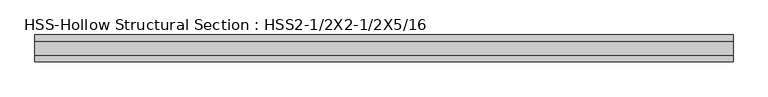
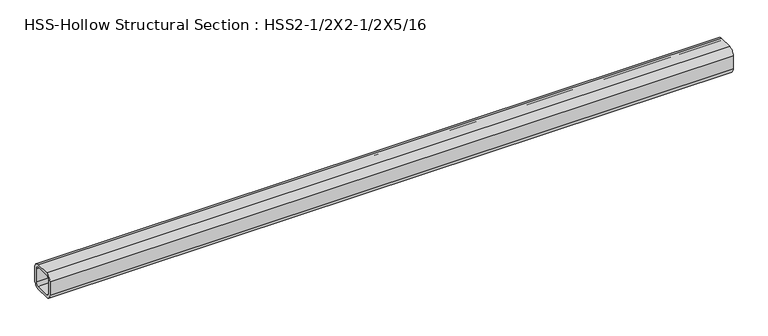
"""IFC4 building model written with IfcOpenShell, lengths in millimetres: beam geometry, HSS-Hollow Structural Section : HSS2-1/2X2-1/2X5/16."""

from ifc_helpers import new_model, si_unit, point, frame, frame_2d, origin, place, context, project, spatial, polyline, circle_curve, trimmed, segment, composite_curve, outline, extrude, source, transform, mapped, element, save


def hss_hollow_structural_section_hss2_1_2x2_1_2x5_16_a2c138a2(model_context):
    return source(origin(), model_context, "Body", "SweptSolid", [
        extrude(outline(composite_curve([segment(polyline([(31.75, 16.9672), (31.75, -16.9672)]), True, "CONTINUOUS"), segment(trimmed(circle_curve(frame_2d((16.9672, -16.9672)), 14.7828), [point((31.75, -16.9672))], [point((16.9672, -31.75))], False, "CARTESIAN"), True, "CONTINUOUS"), segment(polyline([(16.9672, -31.75), (-16.9672, -31.75)]), True, "CONTINUOUS"), segment(trimmed(circle_curve(frame_2d((-16.9672, -16.9672)), 14.7828), [point((-16.9672, -31.75))], [point((-31.75, -16.9672))], False, "CARTESIAN"), True, "CONTINUOUS"), segment(polyline([(-31.75, -16.9672), (-31.75, 16.9672)]), True, "CONTINUOUS"), segment(trimmed(circle_curve(frame_2d((-16.9672, 16.9672)), 14.7828), [point((-31.75, 16.9672))], [point((-16.9672, 31.75))], False, "CARTESIAN"), True, "CONTINUOUS"), segment(polyline([(-16.9672, 31.75), (16.9672, 31.75)]), True, "CONTINUOUS"), segment(trimmed(circle_curve(frame_2d((16.9672, 16.9672)), 14.7828), [point((16.9672, 31.75))], [point((31.75, 16.9672))], False, "CARTESIAN"), True, "CONTINUOUS")], self_intersect=False), holes=[composite_curve([segment(trimmed(circle_curve(frame_2d((-16.9672, 16.9672)), 7.3914), [point((-16.9672, 24.3586))], [point((-24.3586, 16.9672))], True, "CARTESIAN"), True, "CONTINUOUS"), segment(polyline([(-24.3586, 16.9672), (-24.3586, -16.9672)]), True, "CONTINUOUS"), segment(trimmed(circle_curve(frame_2d((-16.9672, -16.9672)), 7.3914), [point((-24.3586, -16.9672))], [point((-16.9672, -24.3586))], True, "CARTESIAN"), True, "CONTINUOUS"), segment(polyline([(-16.9672, -24.3586), (16.9672, -24.3586)]), True, "CONTINUOUS"), segment(trimmed(circle_curve(frame_2d((16.9672, -16.9672)), 7.3914), [point((16.9672, -24.3586))], [point((24.3586, -16.9672))], True, "CARTESIAN"), True, "CONTINUOUS"), segment(polyline([(24.3586, -16.9672), (24.3586, 16.9672)]), True, "CONTINUOUS"), segment(trimmed(circle_curve(frame_2d((16.9672, 16.9672)), 7.3914), [point((24.3586, 16.9672))], [point((16.9672, 24.3586))], True, "CARTESIAN"), True, "CONTINUOUS"), segment(polyline([(16.9672, 24.3586), (-16.9672, 24.3586)]), True, "CONTINUOUS")], self_intersect=False)]), frame((-806.45, 0.0, 0.0), z_axis=(1.0, 0.0, 0.0), x_axis=(0.0, 1.0, 0.0)), (0.0, 0.0, 1.0), 1657.223),
    ])


if __name__ == "__main__":
    model = new_model("IFC4")
    model_context = context("Model", 3, world=origin())
    ifc_project = project(units=[si_unit("LENGTHUNIT", "METRE", prefix="MILLI")], contexts=[model_context])
    site = spatial("IfcSite", under=ifc_project)
    building = spatial("IfcBuilding", under=site)
    placement = place(None, origin())
    hss_hollow_structural_section_hss2_1_2x2_1_2x5_16_shape = hss_hollow_structural_section_hss2_1_2x2_1_2x5_16_a2c138a2(model_context)
    element("IfcBeam", 1, ObjectType="HSS-Hollow Structural Section : HSS2-1/2X2-1/2X5/16", at=placement, inside=building, context=model_context, shape_type="MappedRepresentation", body=[
        mapped(hss_hollow_structural_section_hss2_1_2x2_1_2x5_16_shape, transform((0.0, 0.0, 0.0), x_axis=(1.0, 0.0, 0.0), y_axis=(0.0, 1.0, 0.0), z_axis=(0.0, 0.0, 1.0))),
    ])
    save(model, "model.ifc")

# Revit data of these elements
# Type "HSS-Hollow Structural Section : HSS2-1/2X2-1/2X5/16"
#   Assembly Code = "B10"
#   Shape = "Square"
#   W = 8.4
#   Ht = 0' - 2 1/2"
#   Length [instance default] = 5' - 0"
#   b = 0' - 2 1/2"
#   kr = 0' - 0.582"
#   t = 0' - 0.291"
#   A = 0.0163194 SF
#   Structural Material [instance default] = Steel ASTM A500, Grade B, Rectangular and Square
# Element 1 (IfcBeam, "HSS-Hollow Structural Section : HSS2-1/2X2-1/2X5/16")
#   Materials on its faces: "Steel ASTM A500, Grade B, Rectangular and Square"
# Materials
#   "Steel ASTM A500, Grade B, Rectangular and Square": class "Metal", colour RGB 199 199 199, transparency 0, Description = "Carbon steel", Cost = 0
